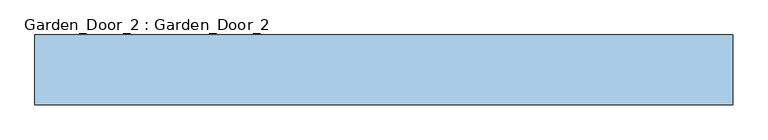
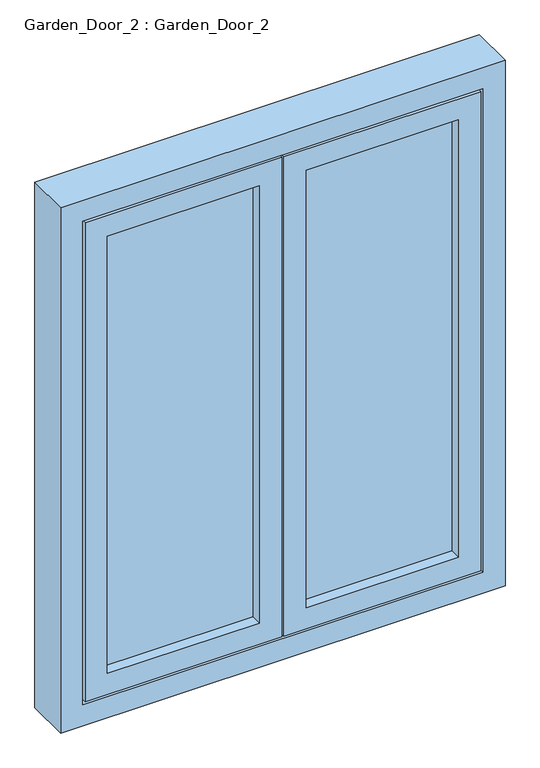
"""IFC4 building model written with IfcOpenShell, lengths in millimetres: window geometry, Garden_Door_2 : Garden_Door_2."""

from ifc_helpers import new_model, si_unit, frame, origin, place, context, project, spatial, polyline, outline, extrude, source, transform, mapped, element, save


def garden_door_2_garden_door_2_d5e40104(model_context):
    return source(origin(), model_context, "Body", "SweptSolid", [
        extrude(outline(polyline([(4115.0, 16765.0), (4800.0, 16765.0), (4800.0, 16755.0), (4115.0, 16755.0), (4115.0, 16765.0)])), frame((0.0, 0.0, 460.0), z_axis=(0.0, 0.0, 1.0), x_axis=(1.0, 0.0, 0.0)), (0.0, 0.0, 1.0), 2080.0),
        extrude(outline(polyline([(360.0, 4900.0), (2640.0, 4900.0), (2640.0, 4015.0), (360.0, 4015.0), (360.0, 4900.0)]), holes=[polyline([(460.0, 4115.0), (2540.0, 4115.0), (2540.0, 4800.0), (460.0, 4800.0), (460.0, 4115.0)])]), frame((0.0, 16705.0, 0.0), z_axis=(0.0, 1.0, 0.0), x_axis=(0.0, 0.0, 1.0)), (0.0, 0.0, 1.0), 100.0),
        extrude(outline(polyline([(3220.0, 16765.0), (3905.0, 16765.0), (3905.0, 16755.0), (3220.0, 16755.0), (3220.0, 16765.0)])), frame((0.0, 0.0, 460.0), z_axis=(0.0, 0.0, 1.0), x_axis=(1.0, 0.0, 0.0)), (0.0, 0.0, 1.0), 2080.0),
        extrude(outline(polyline([(360.0, 4005.0), (2640.0, 4005.0), (2640.0, 3120.0), (360.0, 3120.0), (360.0, 4005.0)]), holes=[polyline([(460.0, 3220.0), (2540.0, 3220.0), (2540.0, 3905.0), (460.0, 3905.0), (460.0, 3220.0)])]), frame((0.0, 16705.0, 0.0), z_axis=(0.0, 1.0, 0.0), x_axis=(0.0, 0.0, 1.0)), (0.0, 0.0, 1.0), 100.0),
        extrude(outline(polyline([(250.0, 5010.0), (2750.0, 5010.0), (2750.0, 3010.0), (250.0, 3010.0), (250.0, 5010.0)]), holes=[polyline([(350.0, 3110.0), (2650.0, 3110.0), (2650.0, 4910.0), (350.0, 4910.0), (350.0, 3110.0)])]), frame((0.0, 16705.0, 0.0), z_axis=(0.0, 1.0, 0.0), x_axis=(0.0, 0.0, 1.0)), (0.0, 0.0, 1.0), 200.0),
    ])


if __name__ == "__main__":
    model = new_model("IFC4")
    model_context = context("Model", 3, world=origin())
    ifc_project = project(units=[si_unit("LENGTHUNIT", "METRE", prefix="MILLI")], contexts=[model_context])
    site = spatial("IfcSite", under=ifc_project)
    building = spatial("IfcBuilding", under=site)
    placement = place(None, origin())
    garden_door_2_garden_door_2_shape = garden_door_2_garden_door_2_d5e40104(model_context)
    element("IfcWindow", 1, ObjectType="Garden_Door_2 : Garden_Door_2", at=placement, inside=building, context=model_context, shape_type="MappedRepresentation", body=[
        mapped(garden_door_2_garden_door_2_shape, transform((0.0, 0.0, 0.0), x_axis=(1.0, 0.0, 0.0), y_axis=(0.0, 1.0, 0.0), z_axis=(0.0, 0.0, 1.0))),
    ])
    save(model, "model.ifc")

# Revit data of these elements
# Type "Garden_Door_2 : Garden_Door_2"
#   Type Mark = "51"
#   NameOverride = "Garden_Door_2"
# Element 1 (IfcWindow, "Garden_Door_2 : Garden_Door_2")
#   Materials on its faces: "IfcSurfaceStyle #392", "IfcSurfaceStyle #398"
# Materials
#   "IfcSurfaceStyle #392": class "Unassigned", colour RGB 204 204 204, transparency 0
#   "IfcSurfaceStyle #398": class "Unassigned", colour RGB 93 183 203, transparency 0.85
